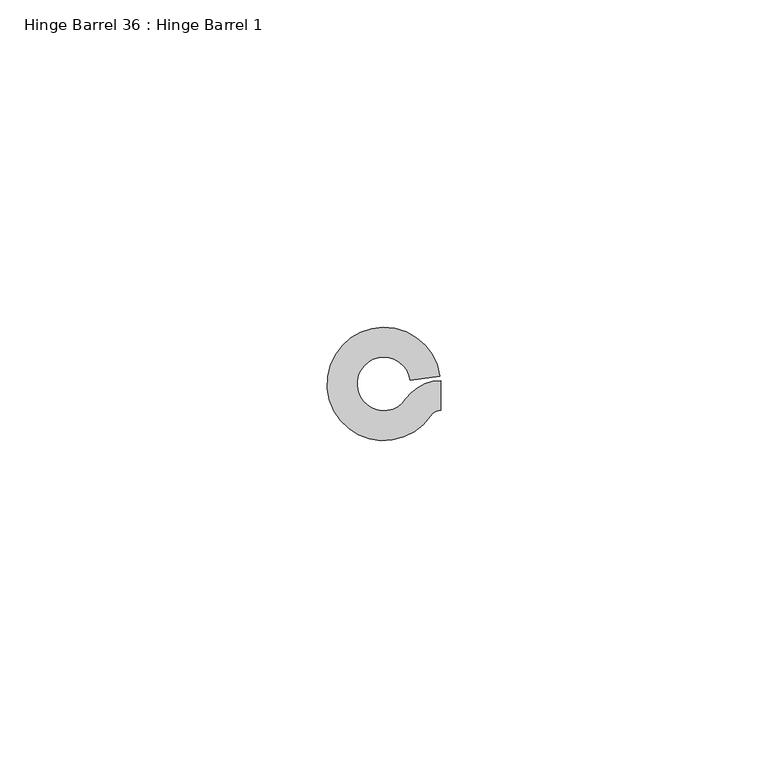
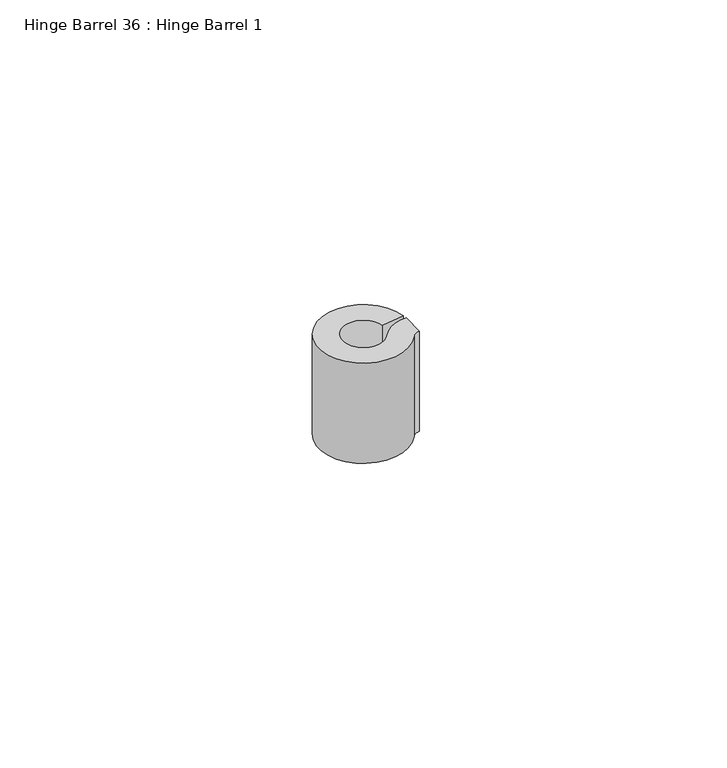
"""IFC4 building model written with IfcOpenShell, lengths in millimetres: proxy geometry, Hinge Barrel 36 : Hinge Barrel 1."""

from ifc_helpers import new_model, si_unit, point, frame, frame_2d, origin, place, context, project, spatial, polyline, circle_curve, trimmed, segment, composite_curve, outline, extrude, source, transform, mapped, element, save


def hinge_barrel_36_hinge_barrel_1_4bd796ae(model_context):
    return source(origin(), model_context, "Body", "SweptSolid", [
        extrude(outline(composite_curve([segment(trimmed(circle_curve(frame_2d((587327.8245257, -533990.5568067)), 6.4044851), [point((587322.5194669, -533986.9688017))], [point((587327.8245257, -533984.1523216))], False, "CARTESIAN"), True, "CONTINUOUS"), segment(polyline([(587327.8245257, -533984.1523216), (587327.8245257, -533988.7163841)]), True, "CONTINUOUS"), segment(trimmed(circle_curve(frame_2d((587327.8245257, -533990.5568067)), 1.8404226), [point((587327.8245257, -533988.7163841))], [point((587326.3000393, -533989.5257409))], True, "CARTESIAN"), True, "CONTINUOUS"), segment(trimmed(circle_curve(frame_2d((587319.1320739, -533984.6777841)), 8.6534625), [point((587326.3000393, -533989.5257409))], [point((587327.7022899, -533983.4803654))], False, "CARTESIAN"), True, "CONTINUOUS"), segment(polyline([(587327.7022899, -533983.4803654), (587323.1821338, -533984.1119153)]), True, "CONTINUOUS"), segment(trimmed(circle_curve(frame_2d((587319.1320739, -533984.6777841)), 4.0894), [point((587323.1821338, -533984.1119153))], [point((587322.5194669, -533986.9688017))], True, "CARTESIAN"), True, "CONTINUOUS")], self_intersect=False)), frame((0.0, 0.0, 1250.95), z_axis=(0.0, 0.0, 1.0), x_axis=(1.0, 0.0, 0.0)), (0.0, 0.0, 1.0), 20.8359375),
    ])


if __name__ == "__main__":
    model = new_model("IFC4")
    model_context = context("Model", 3, world=origin())
    ifc_project = project(units=[si_unit("LENGTHUNIT", "METRE", prefix="MILLI")], contexts=[model_context])
    site = spatial("IfcSite", under=ifc_project)
    building = spatial("IfcBuilding", under=site)
    placement = place(None, origin())
    hinge_barrel_36_hinge_barrel_1_shape = hinge_barrel_36_hinge_barrel_1_4bd796ae(model_context)
    element("IfcBuildingElementProxy", 1, Name="Hinge Barrel 36 : Hinge Barrel 1", ObjectType="Hinge Barrel 36 : Hinge Barrel 1", at=placement, inside=building, context=model_context, shape_type="MappedRepresentation", body=[
        mapped(hinge_barrel_36_hinge_barrel_1_shape, transform((0.0, 0.0, 0.0), x_axis=(1.0, 0.0, 0.0), y_axis=(0.0, 1.0, 0.0), z_axis=(0.0, 0.0, 1.0))),
    ])
    save(model, "model.ifc")

# Revit data of these elements
# Element 1 (IfcBuildingElementProxy, "Hinge Barrel 36 : Hinge Barrel 1")
#   Materials on its faces: "6\"X6\" WELD-ON STL BUTT HINGE"
# Materials
#   "6\"X6\" WELD-ON STL BUTT HINGE": class "Metal", colour RGB 189 187 185, transparency 0, Description = "Carbon steel", Cost = 0
